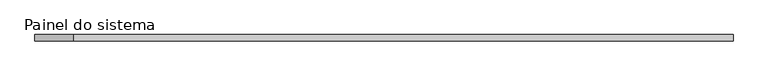
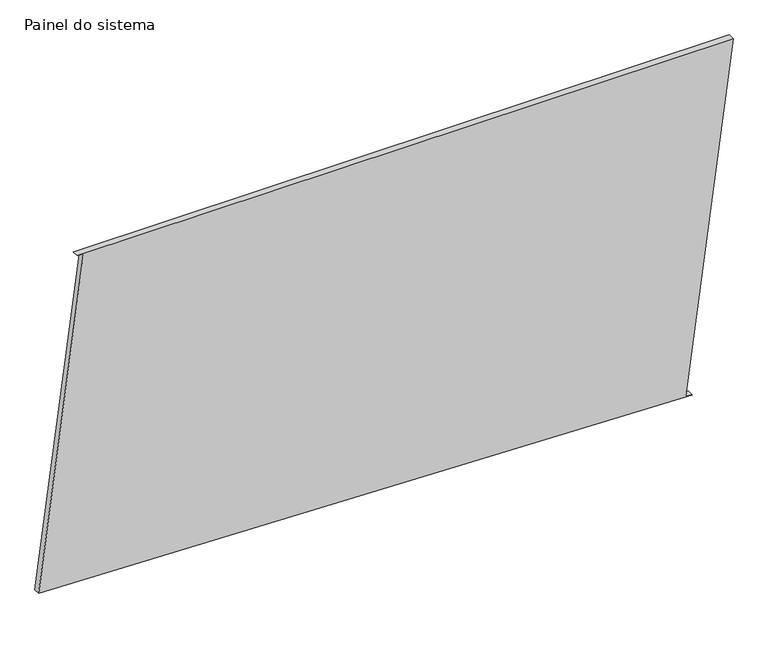
"""IFC4 building model written with IfcOpenShell, lengths in millimetres: plate geometry, Painel do sistema : Envidraçado."""

from ifc_helpers import new_model, si_unit, frame, origin, place, context, project, spatial, polyline, outline, extrude, source, transform, mapped, element, save


def painel_do_sistema_a28059c2(model_context):
    return source(origin(), model_context, "Body", "SweptSolid", [
        extrude(outline(polyline([(0.0, 1199.7403897), (3.2380023, 1174.9509698), (1419.898038, 1359.995574), (1419.898038, -1209.2748481), (1416.6600357, -1184.4854282), (72.9936776, -1359.995574), (0.0, 1199.7403897)])), frame((0.0, 24.5, 0.0), z_axis=(0.0, 1.0, 0.0), x_axis=(0.0, 0.0, 1.0)), (0.0, 0.0, 1.0), 25.0),
    ])


if __name__ == "__main__":
    model = new_model("IFC4")
    model_context = context("Model", 3, world=origin())
    ifc_project = project(units=[si_unit("LENGTHUNIT", "METRE", prefix="MILLI")], contexts=[model_context])
    site = spatial("IfcSite", under=ifc_project)
    building = spatial("IfcBuilding", under=site)
    placement = place(None, origin())
    painel_do_sistema_shape = painel_do_sistema_a28059c2(model_context)
    element("IfcPlate", 1, ObjectType="Painel do sistema : Envidraçado", at=placement, inside=building, context=model_context, shape_type="MappedRepresentation", body=[
        mapped(painel_do_sistema_shape, transform((0.0, 0.0, 0.0), x_axis=(1.0, 0.0, 0.0), y_axis=(0.0, 1.0, 0.0), z_axis=(0.0, 0.0, 1.0))),
    ])
    save(model, "model.ifc")

# Revit data of these elements
# Type "Painel do sistema : Envidraçado"
#   Construction Type Id = "GSP4R"
#   Analytic Construction = "Vidraça única Pilkington 1/8 pol"
#   Visual Light Transmittance = 0.9
#   Solar Heat Gain Coefficient = 0.86
#   Heat Transfer Coefficient (U) = 6.7069 W/(m²·K)
# Element 1 (IfcPlate, "Painel do sistema : Envidraçado")
#   Materials on its faces: "Vidro"
# Materials
#   "Vidro": class "Vidro", colour RGB 0 128 192, transparency 0.9, Description = "Vidro de sílica", Cost = 0
